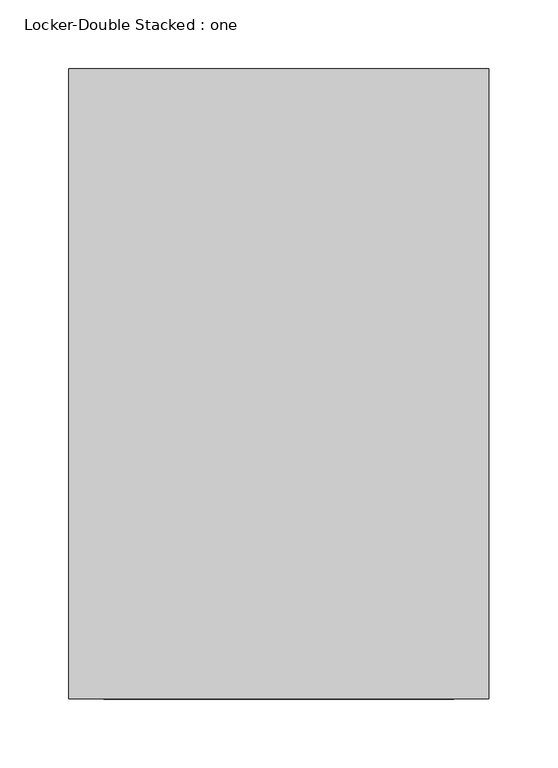
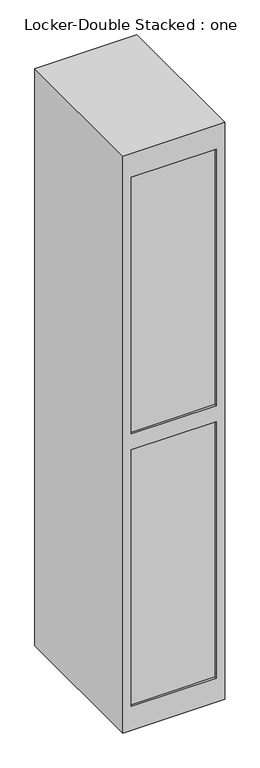
"""IFC4 building model written with IfcOpenShell, lengths in millimetres: furniture geometry, Locker-Double Stacked : one."""

import ifcopenshell
import ifcopenshell.guid

model = None  # the IFC model being written
_history = None  # IfcOwnerHistory: only IFC2X3 demands one
_inside = {}  # id of a spatial element -> (the spatial element, [elements in it])
_under = {}  # id of a project, library or spatial element -> (it, [spatial elements below it])
_declared = {}  # id of a project -> (the project, [libraries it declares])
_typed = {}  # id of a type object -> (the type object, [elements of that type])
_made_of = {}  # id of a material, layer set ... -> (it, [elements and type objects made of it])


def new_model(schema):
    """Start an empty IFC model of exactly this schema.

    Asked for "IFC4X3", IfcOpenShell would pick the latest addendum, in which some entities
    have other attributes; the version numbers below select the first issue.
    IFC2X3 requires an IfcOwnerHistory on every rooted entity: one is made here for all.
    """
    global model, _history
    if schema == "IFC4X3":
        model = ifcopenshell.file(schema_version=(4, 3, 0, 0))
    else:
        model = ifcopenshell.file(schema=schema)
    _inside.clear()
    _under.clear()
    _declared.clear()
    _typed.clear()
    _made_of.clear()
    _history = None
    if model.schema == "IFC2X3":
        org = make("IfcOrganization", Name="unknown")
        user = make(
            "IfcPersonAndOrganization",
            ThePerson=make("IfcPerson", FamilyName="unknown"),
            TheOrganization=org,
        )
        app = make(
            "IfcApplication",
            ApplicationDeveloper=org,
            Version="unknown",
            ApplicationFullName="unknown",
            ApplicationIdentifier="unknown",
        )
        _history = make(
            "IfcOwnerHistory",
            OwningUser=user,
            OwningApplication=app,
            ChangeAction="ADDED",
            CreationDate=0,
        )
    return model


def make(cls, **values):
    """One entity of the class cls with the attributes given. An attribute that is None is left unset."""
    return model.create_entity(
        cls, **{name: value for name, value in values.items() if value is not None}
    )


def rooted(cls, **values):
    """An entity with a GlobalId (a new one), such as an element, a storey or a relation."""
    return make(cls, GlobalId=ifcopenshell.guid.new(), OwnerHistory=_history, **values)


def si_unit(unit_type, name, prefix=None):
    """IfcSIUnit, for example si_unit("LENGTHUNIT", "METRE", prefix="MILLI")."""
    return make("IfcSIUnit", UnitType=unit_type, Prefix=prefix, Name=name)


def assignment(units):
    """IfcUnitAssignment: the units of a project."""
    return None if units is None else make("IfcUnitAssignment", Units=units)


def point(xyz):
    """IfcCartesianPoint."""
    return None if xyz is None else make("IfcCartesianPoint", Coordinates=xyz)


def direction(xyz):
    """IfcDirection."""
    return None if xyz is None else make("IfcDirection", DirectionRatios=xyz)


def frame(location, z_axis=None, x_axis=None):
    """IfcAxis2Placement3D, a coordinate frame: its origin and axes. An axis left out is left unset."""
    return make(
        "IfcAxis2Placement3D",
        Location=point(location),
        Axis=direction(z_axis),
        RefDirection=direction(x_axis),
    )


def origin():
    """The frame at (0, 0, 0) with its axes left unset."""
    return frame((0.0, 0.0, 0.0))


def place(relative_to, where):
    """IfcLocalPlacement: puts the frame where relative to a parent placement (None: the world)."""
    return make(
        "IfcLocalPlacement", PlacementRelTo=relative_to, RelativePlacement=where
    )


def context(
    kind, dimensions, precision=None, world=None, true_north=None, identifier=None
):
    """IfcGeometricRepresentationContext, for example the 3D "Model" context."""
    return make(
        "IfcGeometricRepresentationContext",
        ContextIdentifier=identifier,
        ContextType=kind,
        CoordinateSpaceDimension=dimensions,
        Precision=precision,
        WorldCoordinateSystem=world,
        TrueNorth=true_north,
    )


def project(units=None, contexts=None):
    """IfcProject with its units and contexts."""
    return rooted(
        "IfcProject",
        Name="project",
        RepresentationContexts=contexts,
        UnitsInContext=assignment(units),
    )


def spatial(cls, under=None, at=None, **own):
    """A site, building, storey or space (cls), placed at a placement, below another one or the project."""
    s = rooted(cls, ObjectPlacement=at, **own)
    if under is not None:
        _under.setdefault(under.id(), (under, []))[1].append(s)
    return s


def faces_of(points, faces, orient=None, outer=None):
    """IfcFace entities. A face is a list of loops; a loop is a list of indices into points, from 0.

    orient and outer hold one flag for each loop. By default every Orientation is true, the
    first loop of a face is its IfcFaceOuterBound and the others are IfcFaceBound.
    """
    made = []
    for i, loops in enumerate(faces):
        bounds = []
        for j, loop in enumerate(loops):
            is_outer = j == 0 if outer is None else outer[i][j]
            bounds.append(
                make(
                    "IfcFaceOuterBound" if is_outer else "IfcFaceBound",
                    Bound=make("IfcPolyLoop", Polygon=[points[k] for k in loop]),
                    Orientation=True if orient is None else orient[i][j],
                )
            )
        made.append(make("IfcFace", Bounds=bounds))
    return made


def faceted_brep(points, faces, orient=None, outer=None, voids=None):
    """IfcFacetedBrep: a solid bounded by flat faces; with voids (closed shells), ...WithVoids."""
    shared = [point(p) for p in points]
    hull = make("IfcClosedShell", CfsFaces=faces_of(shared, faces, orient, outer))
    if voids is None:
        return make("IfcFacetedBrep", Outer=hull)
    return make(
        "IfcFacetedBrepWithVoids",
        Outer=hull,
        Voids=[
            make(cls, CfsFaces=faces_of(shared, fs, o, b)) for cls, fs, o, b in voids
        ],
    )


def shape(context_of_items, identifier, shape_type, items):
    """IfcShapeRepresentation: the items that make up one representation, for example the "Body"."""
    return make(
        "IfcShapeRepresentation",
        ContextOfItems=context_of_items,
        RepresentationIdentifier=identifier,
        RepresentationType=shape_type,
        Items=items,
    )


def source(mapping_origin, context_of_items, identifier, shape_type, items):
    """IfcRepresentationMap: a shape defined once, which mapped items show again and again."""
    return make(
        "IfcRepresentationMap",
        MappingOrigin=mapping_origin,
        MappedRepresentation=shape(context_of_items, identifier, shape_type, items),
    )


def transform(
    local_origin,
    x_axis=None,
    y_axis=None,
    z_axis=None,
    scale=None,
    scale2=None,
    scale3=None,
    uniform=True,
):
    """IfcCartesianTransformationOperator3D, or its non-uniform kind. x_axis, y_axis, z_axis: its Axis1, 2, 3."""
    if uniform:
        return make(
            "IfcCartesianTransformationOperator3D",
            Axis1=direction(x_axis),
            Axis2=direction(y_axis),
            LocalOrigin=point(local_origin),
            Scale=scale,
            Axis3=direction(z_axis),
        )
    return make(
        "IfcCartesianTransformationOperator3DnonUniform",
        Axis1=direction(x_axis),
        Axis2=direction(y_axis),
        LocalOrigin=point(local_origin),
        Scale=scale,
        Axis3=direction(z_axis),
        Scale2=scale2,
        Scale3=scale3,
    )


def mapped(mapping_source, mapping_target):
    """IfcMappedItem: shows the shape of a source again, moved by a transform."""
    return make(
        "IfcMappedItem", MappingSource=mapping_source, MappingTarget=mapping_target
    )


def made_of(thing, what):
    """Note that an element or type object is made of a material, layer set ...; save() writes the relation."""
    if what is not None:
        _made_of.setdefault(what.id(), (what, []))[1].append(thing)
    return thing


def element(
    cls,
    number,
    at=None,
    inside=None,
    cuts=None,
    type_object=None,
    material=None,
    context=None,
    identifier="Body",
    shape_type=None,
    held_by="IfcProductDefinitionShape",
    body=None,
    shapes=None,
    **own,
):
    """One element of the class cls, such as IfcWall. Its Tag is "e" and its number.

    at: its placement. inside: the storey or other place that contains it. cuts: it is an
    opening in that element (IfcRelVoidsElement). A single representation is given by context,
    identifier, shape_type and body (its items); several are given by shapes. held_by: the class
    of the entity that holds the representations. save() writes the other relations.
    """
    e = rooted(cls, Tag="e%d" % number, ObjectPlacement=at, **own)
    if body is not None:
        shapes = [shape(context, identifier, shape_type, body)]
    if shapes is not None:
        e.Representation = make(held_by, Representations=shapes)
    if inside is not None:
        _inside.setdefault(inside.id(), (inside, []))[1].append(e)
    if cuts is not None:
        rooted(
            "IfcRelVoidsElement", RelatingBuildingElement=cuts, RelatedOpeningElement=e
        )
    if type_object is not None:
        _typed.setdefault(type_object.id(), (type_object, []))[1].append(e)
    return made_of(e, material)


def aggregate(whole, parts):
    """IfcRelAggregates: a whole, such as a stair, and the parts it consists of."""
    return rooted("IfcRelAggregates", RelatingObject=whole, RelatedObjects=parts)


def save(model, path):
    """Write the relations noted so far, then the file.

    IfcRelAggregates (storeys below a building ...), IfcRelContainedInSpatialStructure (elements
    in a storey), IfcRelDefinesByType, IfcRelAssociatesMaterial and IfcRelDeclares: one each for
    every whole, place, type object, material and project.
    """
    for whole, parts in _under.values():
        aggregate(whole, parts)
    for where, things in _inside.values():
        rooted(
            "IfcRelContainedInSpatialStructure",
            RelatedElements=things,
            RelatingStructure=where,
        )
    for kind, things in _typed.values():
        rooted("IfcRelDefinesByType", RelatedObjects=things, RelatingType=kind)
    for what, things in _made_of.values():
        rooted("IfcRelAssociatesMaterial", RelatedObjects=things, RelatingMaterial=what)
    for by, libraries in _declared.values():
        rooted("IfcRelDeclares", RelatingContext=by, RelatedDefinitions=libraries)
    model.write(path)


def locker_double_stacked_one_5313e0f4(model_context):
    return source(origin(), model_context, "Body", "Brep", [
        faceted_brep([(152.4, -228.6, 1828.8), (152.4, 228.6, 1828.8), (-152.4, 228.6, 1828.8), (-152.4, -228.6, 1828.8), (152.4, -228.6, 0.0), (-152.4, -228.6, 0.0), (-152.4, 228.6, 0.0), (152.4, 228.6, 0.0), (127.0, -228.6, 889.0), (127.0, -228.6, 76.2), (-127.0, -228.6, 76.2), (-127.0, -228.6, 889.0), (-127.0, -228.6, 1752.6), (127.0, -228.6, 1752.6), (127.0, -228.6, 939.8), (-127.0, -228.6, 939.8), (127.0, -222.25, 76.2), (127.0, -222.25, 889.0), (-127.0, -222.25, 889.0), (-127.0, -222.25, 76.2), (127.0, -222.25, 1752.6), (-127.0, -222.25, 1752.6), (-127.0, -222.25, 939.8), (127.0, -222.25, 939.8)], [[[0, 1, 2, 3]], [[4, 5, 6, 7]], [[1, 0, 4, 7]], [[2, 1, 7, 6]], [[3, 2, 6, 5]], [[0, 3, 5, 4], [8, 9, 10, 11], [12, 13, 14, 15]], [[16, 17, 18, 19]], [[17, 16, 9, 8]], [[18, 17, 8, 11]], [[19, 18, 11, 10]], [[16, 19, 10, 9]], [[20, 21, 22, 23]], [[21, 20, 13, 12]], [[22, 21, 12, 15]], [[23, 22, 15, 14]], [[20, 23, 14, 13]]]),
    ])


if __name__ == "__main__":
    model = new_model("IFC4")
    model_context = context("Model", 3, world=origin())
    ifc_project = project(units=[si_unit("LENGTHUNIT", "METRE", prefix="MILLI")], contexts=[model_context])
    site = spatial("IfcSite", under=ifc_project)
    building = spatial("IfcBuilding", under=site)
    placement = place(None, origin())
    locker_double_stacked_one_shape = locker_double_stacked_one_5313e0f4(model_context)
    element("IfcFurniture", 1, ObjectType="Locker-Double Stacked : one", at=placement, inside=building, context=model_context, shape_type="MappedRepresentation", body=[
        mapped(locker_double_stacked_one_shape, transform((0.0, 0.0, 0.0), x_axis=(1.0, 0.0, 0.0), y_axis=(0.0, 1.0, 0.0), z_axis=(0.0, 0.0, 1.0))),
    ])
    save(model, "model.ifc")

# Revit data of these elements
# Type "Locker-Double Stacked : one"
#   Keynote = "M10511300.01"
#   Assembly Code = "E2010"
#   Depth = 1' - 6"
#   Height = 6' - 0"
#   Width = 1' - 0"
#   Material = Metal - Paint Finish - Dark Gray, Matte
# Element 1 (IfcFurniture, "Locker-Double Stacked : one")
#   Materials on its faces: "Metal - Paint Finish - Dark Gray, Matte"
# Materials
#   "Metal - Paint Finish - Dark Gray, Matte": class "Metal", colour RGB 98 98 98, transparency 0
